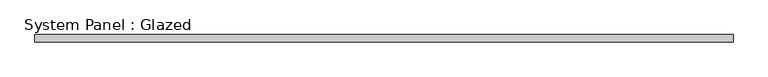
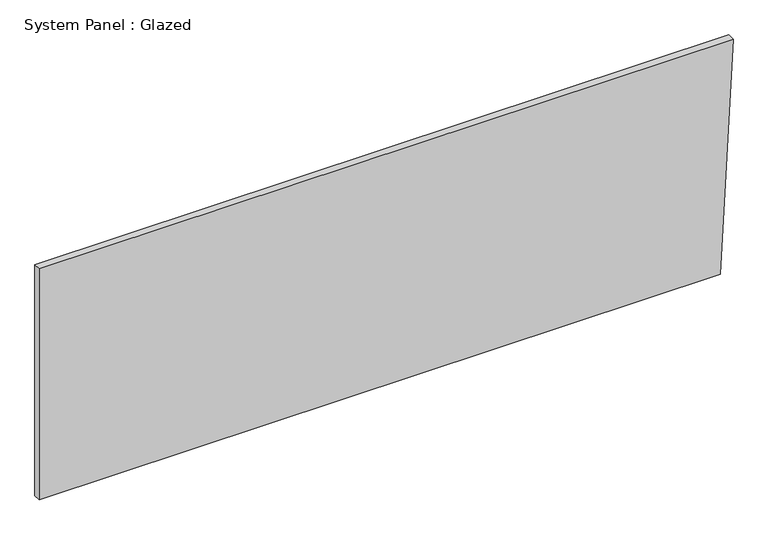
"""IFC4 building model written with IfcOpenShell, lengths in millimetres: plate geometry, System Panel : Glazed."""

from ifc_helpers import new_model, si_unit, frame, origin, place, context, project, spatial, polyline, outline, extrude, source, transform, mapped, element, save


def system_panel_glazed_0a2933fb(model_context):
    return source(origin(), model_context, "Body", "SweptSolid", [
        extrude(outline(polyline([(0.0, -1229.9956829), (0.0, 1184.6684763), (866.081558, 1229.9956829), (866.081558, -1229.9956829), (0.0, -1229.9956829)])), frame((0.0, -44.45, 0.0), z_axis=(0.0, 1.0, 0.0), x_axis=(0.0, 0.0, 1.0)), (0.0, 0.0, 1.0), 25.4),
    ])


if __name__ == "__main__":
    model = new_model("IFC4")
    model_context = context("Model", 3, world=origin())
    ifc_project = project(units=[si_unit("LENGTHUNIT", "METRE", prefix="MILLI")], contexts=[model_context])
    site = spatial("IfcSite", under=ifc_project)
    building = spatial("IfcBuilding", under=site)
    placement = place(None, origin())
    system_panel_glazed_shape = system_panel_glazed_0a2933fb(model_context)
    element("IfcPlate", 1, ObjectType="System Panel : Glazed", at=placement, inside=building, context=model_context, shape_type="MappedRepresentation", body=[
        mapped(system_panel_glazed_shape, transform((0.0, 0.0, 0.0), x_axis=(1.0, 0.0, 0.0), y_axis=(0.0, 1.0, 0.0), z_axis=(0.0, 0.0, 1.0))),
    ])
    save(model, "model.ifc")

# Revit data of these elements
# Type "System Panel : Glazed"
#   Construction Type Id = "GSP4R"
#   Analytic Construction = "1/8 in Pilkington single glazing"
#   Visual Light Transmittance = 0.9
#   Solar Heat Gain Coefficient = 0.86
#   Heat Transfer Coefficient (U) = 1.18115 BTU/(h·ft²·°F)
#   Define Thermal Properties by = 1
# Element 1 (IfcPlate, "System Panel : Glazed")
#   Materials on its faces: "Glass"
# Materials
#   "Glass": class "Glass", colour RGB 0 128 192, transparency 0.75, Description = "Soda Lime Glass", Cost = 0
